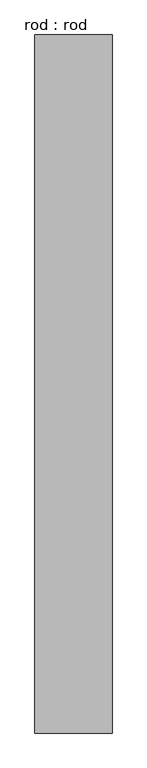
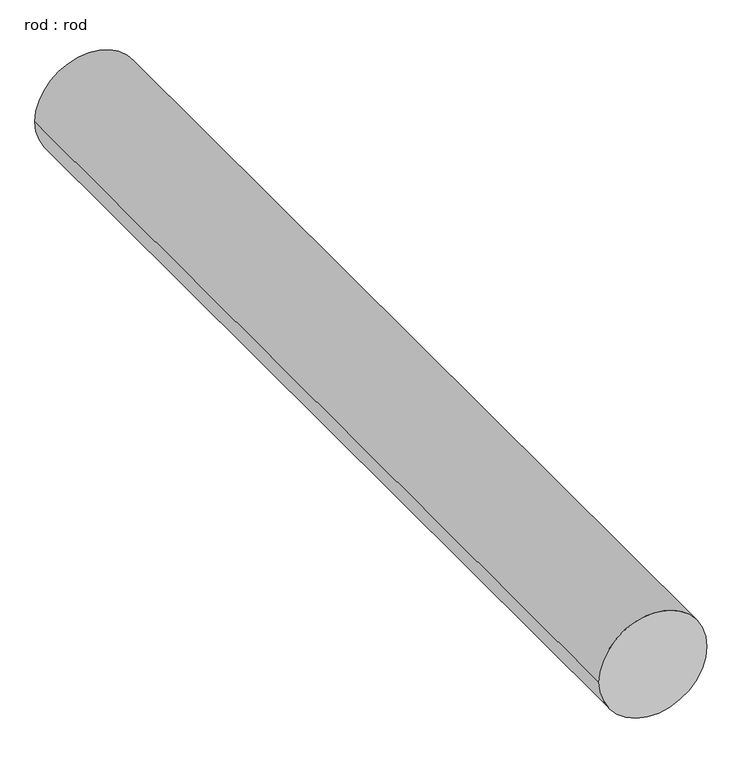
"""IFC4 building model written with IfcOpenShell, lengths in millimetres: proxy geometry, rod : rod."""

from ifc_helpers import new_model, si_unit, point, frame, frame_2d, origin, place, context, project, spatial, circle_curve, trimmed, segment, composite_curve, outline, extrude, source, transform, mapped, element, save


def rod_rod_c8974e2a(model_context):
    return source(origin(), model_context, "Body", "SweptSolid", [
        extrude(outline(composite_curve([segment(trimmed(circle_curve(frame_2d((0.0108462, 0.0)), 200.0), [point((0.0108462, 200.0))], [point((0.0108462, -200.0))], False, "CARTESIAN"), True, "CONTINUOUS"), segment(trimmed(circle_curve(frame_2d((0.0108462, 0.0)), 200.0), [point((0.0108462, -200.0))], [point((0.0108462, 200.0))], False, "CARTESIAN"), True, "CONTINUOUS")], self_intersect=False)), frame((0.0, 2282.326381, 0.0), z_axis=(0.0, 1.0, 0.0), x_axis=(0.0, 0.0, 1.0)), (0.0, 0.0, 1.0), 3620.8044686),
    ])


if __name__ == "__main__":
    model = new_model("IFC4")
    model_context = context("Model", 3, world=origin())
    ifc_project = project(units=[si_unit("LENGTHUNIT", "METRE", prefix="MILLI")], contexts=[model_context])
    site = spatial("IfcSite", under=ifc_project)
    building = spatial("IfcBuilding", under=site)
    placement = place(None, origin())
    rod_rod_shape = rod_rod_c8974e2a(model_context)
    element("IfcBuildingElementProxy", 1, Name="rod : rod", ObjectType="rod : rod", at=placement, inside=building, context=model_context, shape_type="MappedRepresentation", body=[
        mapped(rod_rod_shape, transform((0.0, 0.0, 0.0), x_axis=(1.0, 0.0, 0.0), y_axis=(0.0, 1.0, 0.0), z_axis=(0.0, 0.0, 1.0))),
    ])
    save(model, "model.ifc")

# Revit data of these elements
# Type "rod : rod"
#   Default Elevation = 0
